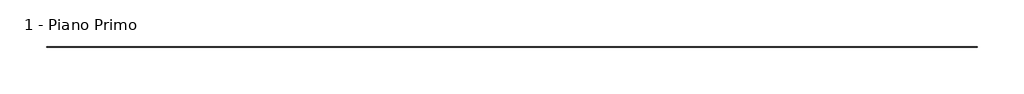
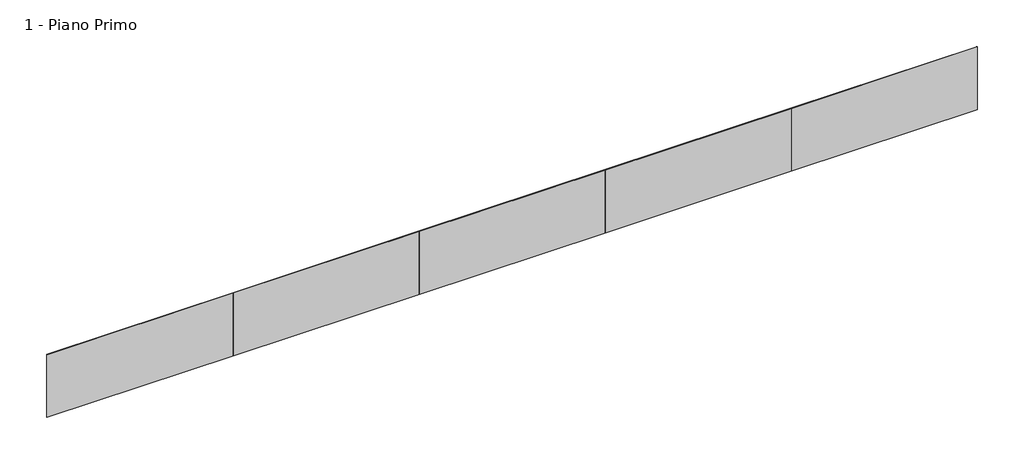
# One storey: 5 plates.
"""IFC4 building model written with IfcOpenShell, lengths in millimetres."""

import ifcopenshell
import ifcopenshell.guid

model = None  # the IFC model being written
_history = None  # IfcOwnerHistory: only IFC2X3 demands one
_inside = {}  # id of a spatial element -> (the spatial element, [elements in it])
_under = {}  # id of a project, library or spatial element -> (it, [spatial elements below it])
_declared = {}  # id of a project -> (the project, [libraries it declares])
_typed = {}  # id of a type object -> (the type object, [elements of that type])
_made_of = {}  # id of a material, layer set ... -> (it, [elements and type objects made of it])


def new_model(schema):
    """Start an empty IFC model of exactly this schema.

    Asked for "IFC4X3", IfcOpenShell would pick the latest addendum, in which some entities
    have other attributes; the version numbers below select the first issue.
    IFC2X3 requires an IfcOwnerHistory on every rooted entity: one is made here for all.
    """
    global model, _history
    if schema == "IFC4X3":
        model = ifcopenshell.file(schema_version=(4, 3, 0, 0))
    else:
        model = ifcopenshell.file(schema=schema)
    _inside.clear()
    _under.clear()
    _declared.clear()
    _typed.clear()
    _made_of.clear()
    _history = None
    if model.schema == "IFC2X3":
        org = make("IfcOrganization", Name="unknown")
        user = make(
            "IfcPersonAndOrganization",
            ThePerson=make("IfcPerson", FamilyName="unknown"),
            TheOrganization=org,
        )
        app = make(
            "IfcApplication",
            ApplicationDeveloper=org,
            Version="unknown",
            ApplicationFullName="unknown",
            ApplicationIdentifier="unknown",
        )
        _history = make(
            "IfcOwnerHistory",
            OwningUser=user,
            OwningApplication=app,
            ChangeAction="ADDED",
            CreationDate=0,
        )
    return model


def make(cls, **values):
    """One entity of the class cls with the attributes given. An attribute that is None is left unset."""
    return model.create_entity(
        cls, **{name: value for name, value in values.items() if value is not None}
    )


def rooted(cls, **values):
    """An entity with a GlobalId (a new one), such as an element, a storey or a relation."""
    return make(cls, GlobalId=ifcopenshell.guid.new(), OwnerHistory=_history, **values)


def si_unit(unit_type, name, prefix=None):
    """IfcSIUnit, for example si_unit("LENGTHUNIT", "METRE", prefix="MILLI")."""
    return make("IfcSIUnit", UnitType=unit_type, Prefix=prefix, Name=name)


def assignment(units):
    """IfcUnitAssignment: the units of a project."""
    return None if units is None else make("IfcUnitAssignment", Units=units)


def point(xyz):
    """IfcCartesianPoint."""
    return None if xyz is None else make("IfcCartesianPoint", Coordinates=xyz)


def direction(xyz):
    """IfcDirection."""
    return None if xyz is None else make("IfcDirection", DirectionRatios=xyz)


def frame(location, z_axis=None, x_axis=None):
    """IfcAxis2Placement3D, a coordinate frame: its origin and axes. An axis left out is left unset."""
    return make(
        "IfcAxis2Placement3D",
        Location=point(location),
        Axis=direction(z_axis),
        RefDirection=direction(x_axis),
    )


def origin():
    """The frame at (0, 0, 0) with its axes left unset."""
    return frame((0.0, 0.0, 0.0))


def origin_with_axes():
    """The frame at (0, 0, 0) with the z axis (0, 0, 1) and the x axis (1, 0, 0) written out."""
    return frame((0.0, 0.0, 0.0), z_axis=(0.0, 0.0, 1.0), x_axis=(1.0, 0.0, 0.0))


def place(relative_to, where):
    """IfcLocalPlacement: puts the frame where relative to a parent placement (None: the world)."""
    return make(
        "IfcLocalPlacement", PlacementRelTo=relative_to, RelativePlacement=where
    )


def context(
    kind, dimensions, precision=None, world=None, true_north=None, identifier=None
):
    """IfcGeometricRepresentationContext, for example the 3D "Model" context."""
    return make(
        "IfcGeometricRepresentationContext",
        ContextIdentifier=identifier,
        ContextType=kind,
        CoordinateSpaceDimension=dimensions,
        Precision=precision,
        WorldCoordinateSystem=world,
        TrueNorth=true_north,
    )


def project(units=None, contexts=None):
    """IfcProject with its units and contexts."""
    return rooted(
        "IfcProject",
        Name="project",
        RepresentationContexts=contexts,
        UnitsInContext=assignment(units),
    )


def spatial(cls, under=None, at=None, **own):
    """A site, building, storey or space (cls), placed at a placement, below another one or the project."""
    s = rooted(cls, ObjectPlacement=at, **own)
    if under is not None:
        _under.setdefault(under.id(), (under, []))[1].append(s)
    return s


def polyline(points):
    """IfcPolyline through the points."""
    return make("IfcPolyline", Points=[point(p) for p in points])


def outline(outer, holes=None, kind="AREA"):
    """IfcArbitraryClosedProfileDef: a profile drawn as a closed curve; with holes, ...WithVoids."""
    if holes is None:
        return make("IfcArbitraryClosedProfileDef", ProfileType=kind, OuterCurve=outer)
    return make(
        "IfcArbitraryProfileDefWithVoids",
        ProfileType=kind,
        OuterCurve=outer,
        InnerCurves=holes,
    )


def extrude(swept, where, along, depth):
    """IfcExtrudedAreaSolid: the profile swept, set in the frame where, extruded along a direction by depth."""
    return make(
        "IfcExtrudedAreaSolid",
        SweptArea=swept,
        Position=where,
        ExtrudedDirection=direction(along),
        Depth=depth,
    )


def shape(context_of_items, identifier, shape_type, items):
    """IfcShapeRepresentation: the items that make up one representation, for example the "Body"."""
    return make(
        "IfcShapeRepresentation",
        ContextOfItems=context_of_items,
        RepresentationIdentifier=identifier,
        RepresentationType=shape_type,
        Items=items,
    )


def source(mapping_origin, context_of_items, identifier, shape_type, items):
    """IfcRepresentationMap: a shape defined once, which mapped items show again and again."""
    return make(
        "IfcRepresentationMap",
        MappingOrigin=mapping_origin,
        MappedRepresentation=shape(context_of_items, identifier, shape_type, items),
    )


def transform(
    local_origin,
    x_axis=None,
    y_axis=None,
    z_axis=None,
    scale=None,
    scale2=None,
    scale3=None,
    uniform=True,
):
    """IfcCartesianTransformationOperator3D, or its non-uniform kind. x_axis, y_axis, z_axis: its Axis1, 2, 3."""
    if uniform:
        return make(
            "IfcCartesianTransformationOperator3D",
            Axis1=direction(x_axis),
            Axis2=direction(y_axis),
            LocalOrigin=point(local_origin),
            Scale=scale,
            Axis3=direction(z_axis),
        )
    return make(
        "IfcCartesianTransformationOperator3DnonUniform",
        Axis1=direction(x_axis),
        Axis2=direction(y_axis),
        LocalOrigin=point(local_origin),
        Scale=scale,
        Axis3=direction(z_axis),
        Scale2=scale2,
        Scale3=scale3,
    )


def mapped(mapping_source, mapping_target):
    """IfcMappedItem: shows the shape of a source again, moved by a transform."""
    return make(
        "IfcMappedItem", MappingSource=mapping_source, MappingTarget=mapping_target
    )


def made_of(thing, what):
    """Note that an element or type object is made of a material, layer set ...; save() writes the relation."""
    if what is not None:
        _made_of.setdefault(what.id(), (what, []))[1].append(thing)
    return thing


def element(
    cls,
    number,
    at=None,
    inside=None,
    cuts=None,
    type_object=None,
    material=None,
    context=None,
    identifier="Body",
    shape_type=None,
    held_by="IfcProductDefinitionShape",
    body=None,
    shapes=None,
    **own,
):
    """One element of the class cls, such as IfcWall. Its Tag is "e" and its number.

    at: its placement. inside: the storey or other place that contains it. cuts: it is an
    opening in that element (IfcRelVoidsElement). A single representation is given by context,
    identifier, shape_type and body (its items); several are given by shapes. held_by: the class
    of the entity that holds the representations. save() writes the other relations.
    """
    e = rooted(cls, Tag="e%d" % number, ObjectPlacement=at, **own)
    if body is not None:
        shapes = [shape(context, identifier, shape_type, body)]
    if shapes is not None:
        e.Representation = make(held_by, Representations=shapes)
    if inside is not None:
        _inside.setdefault(inside.id(), (inside, []))[1].append(e)
    if cuts is not None:
        rooted(
            "IfcRelVoidsElement", RelatingBuildingElement=cuts, RelatedOpeningElement=e
        )
    if type_object is not None:
        _typed.setdefault(type_object.id(), (type_object, []))[1].append(e)
    return made_of(e, material)


def aggregate(whole, parts):
    """IfcRelAggregates: a whole, such as a stair, and the parts it consists of."""
    return rooted("IfcRelAggregates", RelatingObject=whole, RelatedObjects=parts)


def save(model, path):
    """Write the relations noted so far, then the file.

    IfcRelAggregates (storeys below a building ...), IfcRelContainedInSpatialStructure (elements
    in a storey), IfcRelDefinesByType, IfcRelAssociatesMaterial and IfcRelDeclares: one each for
    every whole, place, type object, material and project.
    """
    for whole, parts in _under.values():
        aggregate(whole, parts)
    for where, things in _inside.values():
        rooted(
            "IfcRelContainedInSpatialStructure",
            RelatedElements=things,
            RelatingStructure=where,
        )
    for kind, things in _typed.values():
        rooted("IfcRelDefinesByType", RelatedObjects=things, RelatingType=kind)
    for what, things in _made_of.values():
        rooted("IfcRelAssociatesMaterial", RelatedObjects=things, RelatingMaterial=what)
    for by, libraries in _declared.values():
        rooted("IfcRelDeclares", RelatingContext=by, RelatedDefinitions=libraries)
    model.write(path)


def pannello_sistema_vetrato_29ff3466(model_context):
    return source(origin(), model_context, "Body", "SweptSolid", [
        extrude(outline(polyline([(4200.0000001, -15.0), (-4200.0000001, -15.0), (-4200.0000001, 15.0), (4200.0000001, 15.0), (4200.0000001, -15.0)])), origin_with_axes(), (0.0, 0.0, 1.0), 3000.0),
    ])


model = new_model("IFC4")

# Units and contexts
model_context = context("Model", 3, world=origin())
ifc_project = project(units=[si_unit("LENGTHUNIT", "METRE", prefix="MILLI")], contexts=[model_context])

# Site, building, storey
site = spatial("IfcSite", under=ifc_project)
building = spatial("IfcBuilding", under=site)
storey = spatial("IfcBuildingStorey", under=building, Name="1 - Piano Primo", Elevation=3000.0)

# Plates
placement = place(None, origin())
pannello_sistema_vetrato_shape = pannello_sistema_vetrato_29ff3466(model_context)
element("IfcPlate", 1, ObjectType="Pannello sistema : Vetrato", at=placement, inside=storey, context=model_context, shape_type="MappedRepresentation", body=[
    mapped(pannello_sistema_vetrato_shape, transform((-20934.9893485, 13197.4454735, 3000.0), x_axis=(1.0, 0.0, 0.0), y_axis=(0.0, 1.0, 0.0), z_axis=(0.0, 0.0, 1.0))),
])
element("IfcPlate", 2, ObjectType="Pannello sistema : Vetrato", at=placement, inside=storey, context=model_context, shape_type="MappedRepresentation", body=[
    mapped(pannello_sistema_vetrato_shape, transform((-12534.9893485, 13197.4454735, 3000.0), x_axis=(1.0, 0.0, 0.0), y_axis=(0.0, 1.0, 0.0), z_axis=(0.0, 0.0, 1.0))),
])
element("IfcPlate", 3, ObjectType="Pannello sistema : Vetrato", at=placement, inside=storey, context=model_context, shape_type="MappedRepresentation", body=[
    mapped(pannello_sistema_vetrato_shape, transform((-4134.9893486, 13197.4454735, 3000.0), x_axis=(1.0, 0.0, 0.0), y_axis=(0.0, 1.0, 0.0), z_axis=(0.0, 0.0, 1.0))),
])
element("IfcPlate", 4, ObjectType="Pannello sistema : Vetrato", at=placement, inside=storey, context=model_context, shape_type="MappedRepresentation", body=[
    mapped(pannello_sistema_vetrato_shape, transform((4265.0106513, 13197.4454735, 3000.0), x_axis=(1.0, 0.0, 0.0), y_axis=(0.0, 1.0, 0.0), z_axis=(0.0, 0.0, 1.0))),
])
element("IfcPlate", 5, ObjectType="Pannello sistema : Vetrato", at=placement, inside=storey, context=model_context, shape_type="MappedRepresentation", body=[
    mapped(pannello_sistema_vetrato_shape, transform((12665.0106513, 13197.4454735, 3000.0), x_axis=(1.0, 0.0, 0.0), y_axis=(0.0, 1.0, 0.0), z_axis=(0.0, 0.0, 1.0))),
])

save(model, "model.ifc")

# Revit data of these elements
# Type "Pannello sistema : Vetrato"
#   Construction Type Id = "GSP4R"
#   Analytic Construction = "Vetrata singola Pilkington 1/8 in"
#   Visual Light Transmittance = 0.9
#   Solar Heat Gain Coefficient = 0.86
#   Heat Transfer Coefficient (U) = 6.7069 W/(m²·K)
# Elements 1, 2, 3, 4, 5 (IfcPlate, "Pannello sistema : Vetrato")
#   Phase Created = Stato di Progetto
#   Materials on its faces: "Default - Vetro"
# Materials
#   "Default - Vetro": class "Vetro", colour RGB 208 208 208, transparency 0.7, Cost = 0
